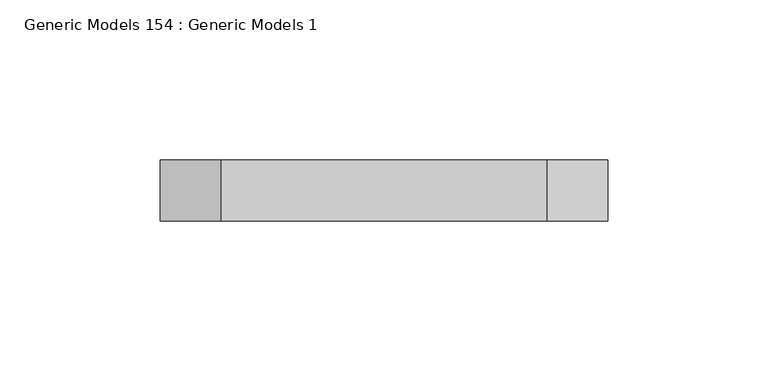
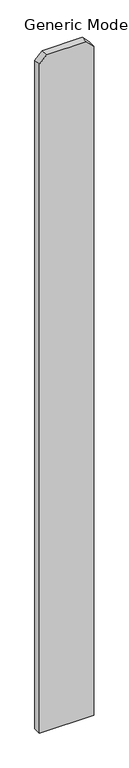
"""IFC4 building model written with IfcOpenShell, lengths in millimetres: proxy geometry, Generic Models 154 : Generic Models 1."""

from ifc_helpers import new_model, si_unit, frame, origin, place, context, project, spatial, polyline, outline, extrude, source, transform, mapped, element, save


def generic_models_154_generic_models_1_356fbd50(model_context):
    return source(origin(), model_context, "Body", "SweptSolid", [
        extrude(outline(polyline([(76.2, -250877.3875), (1885.95, -250877.3875), (1905.0, -250896.4375), (1905.0, -250998.0375), (1885.95, -251017.0875), (76.2, -251017.0875), (76.2, -250877.3875)])), frame((0.0, 547.6875, 0.0), z_axis=(0.0, 1.0, 0.0), x_axis=(0.0, 0.0, 1.0)), (0.0, 0.0, 1.0), 19.05),
    ])


if __name__ == "__main__":
    model = new_model("IFC4")
    model_context = context("Model", 3, world=origin())
    ifc_project = project(units=[si_unit("LENGTHUNIT", "METRE", prefix="MILLI")], contexts=[model_context])
    site = spatial("IfcSite", under=ifc_project)
    building = spatial("IfcBuilding", under=site)
    placement = place(None, origin())
    generic_models_154_generic_models_1_shape = generic_models_154_generic_models_1_356fbd50(model_context)
    element("IfcBuildingElementProxy", 1, Name="Generic Models 154 : Generic Models 1", ObjectType="Generic Models 154 : Generic Models 1", at=placement, inside=building, context=model_context, shape_type="MappedRepresentation", body=[
        mapped(generic_models_154_generic_models_1_shape, transform((0.0, 0.0, 0.0), x_axis=(1.0, 0.0, 0.0), y_axis=(0.0, 1.0, 0.0), z_axis=(0.0, 0.0, 1.0))),
    ])
    save(model, "model.ifc")

# Revit data of these elements
# Element 1 (IfcBuildingElementProxy, "Generic Models 154 : Generic Models 1")
#   Materials on its faces: "VERTICAL 1X6 CEDAR PLANKS W/ CLEAR WOOD SEALER"
# Materials
#   "VERTICAL 1X6 CEDAR PLANKS W/ CLEAR WOOD SEALER": class "Wood", colour RGB 234 198 147, transparency 0, Description = "Pinus Echinata", Cost = 0
